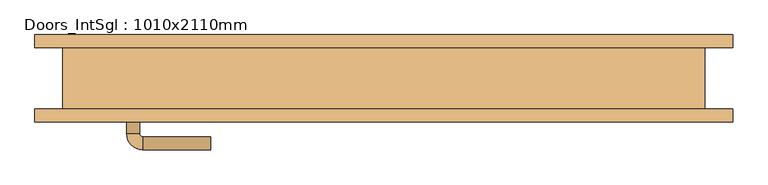
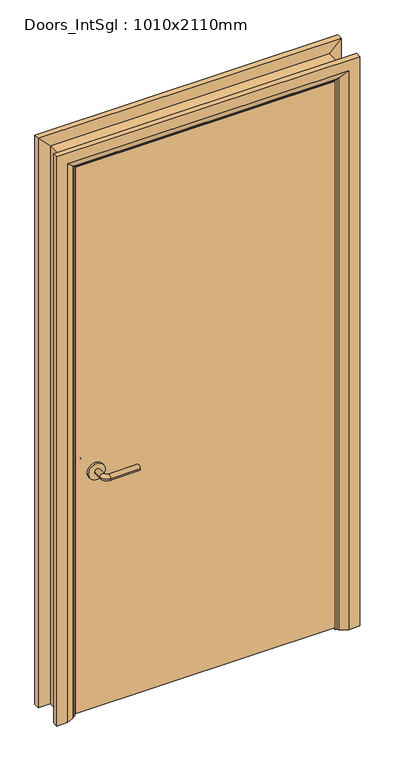
"""IFC4 building model written with IfcOpenShell, lengths in millimetres: door geometry, Doors_IntSgl : 1010x2110mm."""

from ifc_helpers import new_model, si_unit, point, frame, frame_2d, origin, place, context, project, spatial, polyline, circle_curve, ellipse_curve, trimmed, segment, composite_curve, outline, extrude, faceted_brep, source, transform, mapped, element, save
from ifc_brep_helpers import plane_surface, cylinder_surface, revolved_surface, advanced_brep


def doors_intsgl_1010x2110mm_25c8a350(model_context):
    return source(origin(), model_context, "Body", "SolidModel", [
        advanced_brep(
        [(-398.0, -1.5, 900.0), (-378.0, -1.5, 900.0), (-398.0, 28.5, 900.0), (-378.0, 28.5, 900.0), (-373.0, 33.5, 900.0), (-373.0, 53.5, 900.0), (-268.0, 53.5, 900.0), (-268.0, 33.5, 900.0)],
        [
            (0, 1, circle_curve(frame((-388.0, -1.5, 900.0), z_axis=(0.0, -1.0, 0.0), x_axis=(1.0, 0.0, 0.0)), 10.0)),
            (1, 0, circle_curve(frame((-388.0, -1.5, 900.0), z_axis=(0.0, -1.0, 0.0), x_axis=(1.0, 0.0, 0.0)), 10.0)),
            (0, 2),
            (2, 3, circle_curve(frame((-388.0, 28.5, 900.0), z_axis=(0.0, -1.0, 0.0), x_axis=(1.0, 0.0, 0.0)), 10.0)),
            (3, 1),
            (3, 2, circle_curve(frame((-388.0, 28.5, 900.0), z_axis=(0.0, -1.0, 0.0), x_axis=(1.0, 0.0, 0.0)), 10.0)),
            (4, 3, circle_curve(frame((-373.0, 28.5, 900.0), z_axis=(0.0, 0.0, 1.0), x_axis=(-1.0, 0.0, 0.0)), 5.0)),
            (2, 5, circle_curve(frame((-373.0, 28.5, 900.0), z_axis=(0.0, 0.0, -1.0), x_axis=(-1.0, 0.0, 0.0)), 25.0)),
            (5, 4, circle_curve(frame((-373.0, 43.5, 900.0), z_axis=(-1.0, 0.0, 0.0), x_axis=(0.0, -1.0, 0.0)), 10.0)),
            (4, 5, circle_curve(frame((-373.0, 43.5, 900.0), z_axis=(-1.0, 0.0, 0.0), x_axis=(0.0, -1.0, 0.0)), 10.0)),
            (6, 7, circle_curve(frame((-268.0, 43.5, 900.0), z_axis=(1.0, 0.0, 0.0), x_axis=(0.0, -1.0, 0.0)), 10.0)),
            (7, 6, circle_curve(frame((-268.0, 43.5, 900.0), z_axis=(1.0, 0.0, 0.0), x_axis=(0.0, -1.0, 0.0)), 10.0)),
            (5, 6),
            (7, 4),
        ],
        [
            plane_surface(frame((-388.0, -1.5, 900.0), z_axis=(0.0, -1.0, 0.0), x_axis=(0.0, 0.0, 1.0))),
            cylinder_surface(frame((-388.0, -1.5, 900.0), z_axis=(0.0, -1.0, 0.0), x_axis=(1.0, 0.0, 0.0)), 10.0),
            revolved_surface(trimmed(ellipse_curve(frame((-388.0, 28.5, 900.0), z_axis=(0.0, -1.0, 0.0), x_axis=(1.0, 0.0, 0.0)), 10.0, 10.0), [point((-398.0, 28.5, 900.0))], [point((-378.0, 28.5, 900.0))], True, "CARTESIAN"), (-373.0, 28.5, 900.0), (0.0, 0.0, -1.0)),
            revolved_surface(trimmed(ellipse_curve(frame((-388.0, 28.5, 900.0), z_axis=(0.0, -1.0, 0.0), x_axis=(1.0, 0.0, 0.0)), 10.0, 10.0), [point((-378.0, 28.5, 900.0))], [point((-398.0, 28.5, 900.0))], True, "CARTESIAN"), (-373.0, 28.5, 900.0), (0.0, 0.0, -1.0)),
            plane_surface(frame((-268.0, 43.5, 900.0), z_axis=(1.0, 0.0, 0.0), x_axis=(0.0, 0.0, 1.0))),
            cylinder_surface(frame((-373.0, 43.5, 900.0), z_axis=(-1.0, 0.0, 0.0), x_axis=(0.0, -1.0, 0.0)), 10.0),
        ],
        [
            (0, [[1, 2]]),
            (1, [[-1, 3, 4, 5]]),
            (1, [[-2, -5, 6, -3]]),
            (2, [[7, -4, 8, 9]]),
            (3, [[-8, -6, -7, 10]]),
            (4, [[11, 12]]),
            (5, [[-9, 13, -12, 14]]),
            (5, [[-10, -14, -11, -13]]),
        ],
    ),
        extrude(outline(composite_curve([segment(trimmed(circle_curve(frame_2d((900.0, -390.5)), 30.0), [point((900.0, -420.5))], [point((900.0, -360.5))], False, "CARTESIAN"), True, "CONTINUOUS"), segment(trimmed(circle_curve(frame_2d((900.0, -390.5)), 30.0), [point((900.0, -360.5))], [point((900.0, -420.5))], False, "CARTESIAN"), True, "CONTINUOUS")], self_intersect=False)), frame((0.0, -9.5, 0.0), z_axis=(0.0, 1.0, 0.0), x_axis=(0.0, 0.0, 1.0)), (0.0, 0.0, 1.0), 8.0),
        advanced_brep(
        [(-398.0, -55.5, 900.0), (-378.0, -55.5, 900.0), (-378.0, -85.5, 900.0), (-398.0, -85.5, 900.0), (-373.0, -90.5, 900.0), (-373.0, -110.5, 900.0), (-268.0, -110.5, 900.0), (-268.0, -90.5, 900.0)],
        [
            (0, 1, circle_curve(frame((-388.0, -55.5, 900.0), z_axis=(0.0, 1.0, 0.0), x_axis=(1.0, 0.0, 0.0)), 10.0)),
            (1, 0, circle_curve(frame((-388.0, -55.5, 900.0), z_axis=(0.0, 1.0, 0.0), x_axis=(1.0, 0.0, 0.0)), 10.0)),
            (1, 2),
            (2, 3, circle_curve(frame((-388.0, -85.5, 900.0), z_axis=(0.0, 1.0, 0.0), x_axis=(1.0, 0.0, 0.0)), 10.0)),
            (3, 0),
            (3, 2, circle_curve(frame((-388.0, -85.5, 900.0), z_axis=(0.0, 1.0, 0.0), x_axis=(1.0, 0.0, 0.0)), 10.0)),
            (4, 5, circle_curve(frame((-373.0, -100.5, 900.0), z_axis=(-1.0, 0.0, 0.0), x_axis=(0.0, 1.0, 0.0)), 10.0)),
            (5, 3, circle_curve(frame((-373.0, -85.5, 900.0), z_axis=(0.0, 0.0, -1.0), x_axis=(-1.0, 0.0, 0.0)), 25.0)),
            (2, 4, circle_curve(frame((-373.0, -85.5, 900.0), z_axis=(0.0, 0.0, 1.0), x_axis=(-1.0, 0.0, 0.0)), 5.0)),
            (5, 4, circle_curve(frame((-373.0, -100.5, 900.0), z_axis=(-1.0, 0.0, 0.0), x_axis=(0.0, 1.0, 0.0)), 10.0)),
            (6, 7, circle_curve(frame((-268.0, -100.5, 900.0), z_axis=(1.0, 0.0, 0.0), x_axis=(0.0, 1.0, 0.0)), 10.0)),
            (7, 6, circle_curve(frame((-268.0, -100.5, 900.0), z_axis=(1.0, 0.0, 0.0), x_axis=(0.0, 1.0, 0.0)), 10.0)),
            (4, 7),
            (6, 5),
        ],
        [
            plane_surface(frame((-388.0, -55.5, 900.0), z_axis=(0.0, 1.0, 0.0), x_axis=(0.0, 0.0, 1.0))),
            cylinder_surface(frame((-388.0, -55.5, 900.0), z_axis=(0.0, 1.0, 0.0), x_axis=(1.0, 0.0, 0.0)), 10.0),
            revolved_surface(trimmed(ellipse_curve(frame((-388.0, -85.5, 900.0), z_axis=(0.0, -1.0, 0.0), x_axis=(1.0, 0.0, 0.0)), 10.0, 10.0), [point((-398.0, -85.5, 900.0))], [point((-378.0, -85.5, 900.0))], True, "CARTESIAN"), (-373.0, -85.5, 900.0), (0.0, 0.0, -1.0)),
            revolved_surface(trimmed(ellipse_curve(frame((-388.0, -85.5, 900.0), z_axis=(0.0, -1.0, 0.0), x_axis=(1.0, 0.0, 0.0)), 10.0, 10.0), [point((-378.0, -85.5, 900.0))], [point((-398.0, -85.5, 900.0))], True, "CARTESIAN"), (-373.0, -85.5, 900.0), (0.0, 0.0, -1.0)),
            plane_surface(frame((-268.0, -100.5, 900.0), z_axis=(1.0, 0.0, 0.0), x_axis=(0.0, 0.0, 1.0))),
            cylinder_surface(frame((-373.0, -100.5, 900.0), z_axis=(-1.0, 0.0, 0.0), x_axis=(0.0, 1.0, 0.0)), 10.0),
        ],
        [
            (0, [[1, 2]]),
            (1, [[3, 4, 5, -2]]),
            (1, [[-5, 6, -3, -1]]),
            (2, [[7, 8, -4, 9]]),
            (3, [[10, -9, -6, -8]]),
            (4, [[11, 12]]),
            (5, [[13, -11, 14, -7]]),
            (5, [[-14, -12, -13, -10]]),
        ],
    ),
        extrude(outline(composite_curve([segment(trimmed(circle_curve(frame_2d((900.0, -390.5)), 30.0), [point((900.0, -420.5))], [point((900.0, -360.5))], False, "CARTESIAN"), True, "CONTINUOUS"), segment(trimmed(circle_curve(frame_2d((900.0, -390.5)), 30.0), [point((900.0, -360.5))], [point((900.0, -420.5))], False, "CARTESIAN"), True, "CONTINUOUS")], self_intersect=False)), frame((0.0, -55.5, 0.0), z_axis=(0.0, 1.0, 0.0), x_axis=(0.0, 0.0, 1.0)), (0.0, 0.0, 1.0), 8.0),
        extrude(outline(polyline([(463.0, -9.5), (463.0, -47.5), (-463.0, -47.5), (-463.0, -9.5), (463.0, -9.5)])), frame((0.0, 0.0, 8.0), z_axis=(0.0, 0.0, 1.0), x_axis=(1.0, 0.0, 0.0)), (0.0, 0.0, 1.0), 2060.0),
        advanced_brep(
        [(540.0, -67.5, 0.0), (500.0, -67.5, 0.0), (474.0, -53.5, 0.0), (470.0, -47.5, 0.0), (540.0, -47.5, 0.0), (540.0, -47.5, 2145.0), (540.0, -67.5, 2145.0), (470.0, -47.5, 2075.0), (-470.0, -47.5, 2075.0), (-470.0, -47.5, 0.0), (-540.0, -47.5, 0.0), (-540.0, -47.5, 2145.0), (474.0, -53.5, 2079.0), (500.0, -67.5, 2105.0), (-540.0, -67.5, 2145.0), (-540.0, -67.5, 0.0), (-500.0, -67.5, 0.0), (-500.0, -67.5, 2105.0), (-474.0, -53.5, 2079.0), (-474.0, -53.5, 0.0)],
        [
            (0, 1),
            (1, 2),
            (2, 3, circle_curve(frame((478.0, -46.5, 0.0), z_axis=(0.0, 0.0, -1.0), x_axis=(1.0, 0.0, 0.0)), 8.0622577)),
            (3, 4),
            (4, 0),
            (4, 5),
            (5, 6),
            (6, 0),
            (3, 7),
            (7, 8),
            (8, 9),
            (9, 10),
            (10, 11),
            (11, 5),
            (2, 12),
            (12, 7, ellipse_curve(frame((478.0, -46.5, 2083.0), z_axis=(0.7071067811865475, 0.0, -0.7071067811865475), x_axis=(-0.7071067811865474, 0.0, -0.7071067811865476)), 11.4017543, 8.0622577)),
            (1, 13),
            (13, 12),
            (6, 14),
            (14, 15),
            (15, 16),
            (16, 17),
            (17, 13),
            (11, 14),
            (12, 18),
            (18, 8, ellipse_curve(frame((-478.0, -46.5, 2083.0), z_axis=(0.7071067811865475, 0.0, 0.7071067811865475), x_axis=(0.7071067811865476, 0.0, -0.7071067811865474)), 11.4017543, 8.0622577)),
            (17, 18),
            (15, 10),
            (9, 19, circle_curve(frame((-478.0, -46.5, 0.0), z_axis=(0.0, 0.0, -1.0), x_axis=(-1.0, 0.0, 0.0)), 8.0622577)),
            (19, 16),
            (18, 19),
        ],
        [
            plane_surface(frame((470.0, -47.5, 0.0), z_axis=(0.0, 0.0, -1.0), x_axis=(0.0, 1.0, 0.0))),
            plane_surface(frame((540.0, -67.5, 0.0), z_axis=(1.0, 0.0, 0.0), x_axis=(0.0, 0.0, 1.0))),
            plane_surface(frame((540.0, -47.5, 0.0), z_axis=(0.0, 1.0, 0.0), x_axis=(0.0, 0.0, 1.0))),
            cylinder_surface(frame((478.0, -46.5, 0.0), z_axis=(0.0, 0.0, -1.0), x_axis=(1.0, 0.0, 0.0)), 8.0622577),
            plane_surface(frame((474.0, -53.5, 0.0), z_axis=(-0.4740998230350126, -0.880471099922178, 0.0), x_axis=(0.0, 0.0, 1.0))),
            plane_surface(frame((500.0, -67.5, 0.0), z_axis=(0.0, -1.0, 0.0), x_axis=(0.0, 0.0, 1.0))),
            plane_surface(frame((540.0, -67.5, 2145.0), z_axis=(0.0, 0.0, 1.0), x_axis=(-1.0, 0.0, 0.0))),
            cylinder_surface(frame((470.0, -46.5, 2083.0), z_axis=(1.0, 0.0, 0.0), x_axis=(0.0, 0.0, 1.0)), 8.0622577),
            plane_surface(frame((474.0, -53.5, 2079.0), z_axis=(0.0, -0.8804710999221764, -0.4740998230350154), x_axis=(-1.0, 0.0, 0.0))),
            plane_surface(frame((-470.0, -47.5, 0.0), z_axis=(0.0, 0.0, -1.0), x_axis=(0.0, 1.0, 0.0))),
            plane_surface(frame((-540.0, -67.5, 2145.0), z_axis=(-1.0, 0.0, 0.0), x_axis=(0.0, 0.0, -1.0))),
            cylinder_surface(frame((-478.0, -46.5, 2075.0), z_axis=(0.0, 0.0, 1.0), x_axis=(-1.0, 0.0, 0.0)), 8.0622577),
            plane_surface(frame((-474.0, -53.5, 2079.0), z_axis=(0.47409982303501824, -0.8804710999221749, 0.0), x_axis=(0.0, 0.0, -1.0))),
        ],
        [
            (0, [[1, 2, 3, 4, 5]]),
            (1, [[6, 7, 8, -5]]),
            (2, [[9, 10, 11, 12, 13, 14, -6, -4]]),
            (3, [[15, 16, -9, -3]]),
            (4, [[17, 18, -15, -2]]),
            (5, [[-8, 19, 20, 21, 22, 23, -17, -1]]),
            (6, [[-14, 24, -19, -7]]),
            (7, [[25, 26, -10, -16]]),
            (8, [[-23, 27, -25, -18]]),
            (9, [[28, -12, 29, 30, -21]]),
            (10, [[-13, -28, -20, -24]]),
            (11, [[31, -29, -11, -26]]),
            (12, [[-22, -30, -31, -27]]),
        ],
    ),
        extrude(outline(polyline([(0.0, -446.0), (2051.0, -446.0), (2051.0, 446.0), (0.0, 446.0), (0.0, 465.0), (2070.0, 465.0), (2070.0, -465.0), (0.0, -465.0), (0.0, -446.0)])), frame((0.0, -7.5, 0.0), z_axis=(0.0, 1.0, 0.0), x_axis=(0.0, 0.0, 1.0)), (0.0, 0.0, 1.0), 32.0),
        advanced_brep(
        [(-540.0, 67.5, 0.0), (-500.0, 67.5, 0.0), (-474.0, 53.5, 0.0), (-470.0, 47.5, 0.0), (-540.0, 47.5, 0.0), (-540.0, 47.5, 2145.0), (-540.0, 67.5, 2145.0), (-470.0, 47.5, 2075.0), (-474.0, 53.5, 2079.0), (-500.0, 67.5, 2105.0), (540.0, 47.5, 2145.0), (540.0, 67.5, 2145.0), (470.0, 47.5, 2075.0), (474.0, 53.5, 2079.0), (500.0, 67.5, 2105.0), (540.0, 67.5, 0.0), (540.0, 47.5, 0.0), (470.0, 47.5, 0.0), (474.0, 53.5, 0.0), (500.0, 67.5, 0.0)],
        [
            (0, 1),
            (1, 2),
            (2, 3, circle_curve(frame((-478.0, 46.5, 0.0), z_axis=(0.0, 0.0, -1.0), x_axis=(-1.0, 0.0, 0.0)), 8.0622577)),
            (3, 4),
            (4, 0),
            (4, 5),
            (5, 6),
            (6, 0),
            (3, 7),
            (7, 5),
            (2, 8),
            (8, 7, ellipse_curve(frame((-478.0, 46.5, 2083.0), z_axis=(-0.7071067811865475, 0.0, -0.7071067811865475), x_axis=(0.7071067811865474, 0.0, -0.7071067811865476)), 11.4017543, 8.0622577)),
            (1, 9),
            (9, 8),
            (6, 9),
            (5, 10),
            (10, 11),
            (11, 6),
            (7, 12),
            (12, 10),
            (8, 13),
            (13, 12, ellipse_curve(frame((478.0, 46.5, 2083.0), z_axis=(-0.7071067811865475, 0.0, 0.7071067811865475), x_axis=(-0.7071067811865476, 0.0, -0.7071067811865474)), 11.4017543, 8.0622577)),
            (9, 14),
            (14, 13),
            (11, 14),
            (15, 16),
            (16, 17),
            (17, 18, circle_curve(frame((478.0, 46.5, 0.0), z_axis=(0.0, 0.0, -1.0), x_axis=(1.0, 0.0, 0.0)), 8.0622577)),
            (18, 19),
            (19, 15),
            (10, 16),
            (15, 11),
            (12, 17),
            (13, 18),
            (14, 19),
        ],
        [
            plane_surface(frame((-470.0, 120.3010989, 0.0), z_axis=(0.0, 0.0, -1.0), x_axis=(1.0, 0.0, 0.0))),
            plane_surface(frame((-540.0, 67.5, 0.0), z_axis=(-1.0, 0.0, 0.0), x_axis=(0.0, 0.0, 1.0))),
            plane_surface(frame((-540.0, 47.5, 0.0), z_axis=(0.0, -1.0, 0.0), x_axis=(0.0, 0.0, 1.0))),
            cylinder_surface(frame((-478.0, 46.5, 0.0), z_axis=(0.0, 0.0, -1.0), x_axis=(-1.0, 0.0, 0.0)), 8.0622577),
            plane_surface(frame((-474.0, 53.5, 0.0), z_axis=(0.4740998230350183, 0.8804710999221749, 0.0), x_axis=(0.0, 0.0, 1.0))),
            plane_surface(frame((-500.0, 67.5, 0.0), z_axis=(0.0, 1.0, 0.0), x_axis=(0.0, 0.0, 1.0))),
            plane_surface(frame((-540.0, 67.5, 2145.0), z_axis=(0.0, 0.0, 1.0), x_axis=(1.0, 0.0, 0.0))),
            plane_surface(frame((-540.0, 47.5, 2145.0), z_axis=(0.0, -1.0, 0.0), x_axis=(1.0, 0.0, 0.0))),
            cylinder_surface(frame((-470.0, 46.5, 2083.0), z_axis=(-1.0, 0.0, 0.0), x_axis=(0.0, 0.0, 1.0)), 8.0622577),
            plane_surface(frame((-474.0, 53.5, 2079.0), z_axis=(0.0, 0.8804710999221749, -0.4740998230350183), x_axis=(1.0, 0.0, 0.0))),
            plane_surface(frame((-500.0, 67.5, 2105.0), z_axis=(0.0, 1.0, 0.0), x_axis=(1.0, 0.0, 0.0))),
            plane_surface(frame((470.0, 120.3010989, 0.0), z_axis=(0.0, 0.0, -1.0), x_axis=(-1.0, 0.0, 0.0))),
            plane_surface(frame((540.0, 67.5, 2145.0), z_axis=(1.0, 0.0, 0.0), x_axis=(0.0, 0.0, -1.0))),
            plane_surface(frame((540.0, 47.5, 2145.0), z_axis=(0.0, -1.0, 0.0), x_axis=(0.0, 0.0, -1.0))),
            cylinder_surface(frame((478.0, 46.5, 2075.0), z_axis=(0.0, 0.0, 1.0), x_axis=(1.0, 0.0, 0.0)), 8.0622577),
            plane_surface(frame((474.0, 53.5, 2079.0), z_axis=(-0.4740998230350183, 0.8804710999221749, 0.0), x_axis=(0.0, 0.0, -1.0))),
            plane_surface(frame((500.0, 67.5, 2105.0), z_axis=(0.0, 1.0, 0.0), x_axis=(0.0, 0.0, -1.0))),
        ],
        [
            (0, [[1, 2, 3, 4, 5]]),
            (1, [[6, 7, 8, -5]]),
            (2, [[9, 10, -6, -4]]),
            (3, [[11, 12, -9, -3]]),
            (4, [[13, 14, -11, -2]]),
            (5, [[-8, 15, -13, -1]]),
            (6, [[16, 17, 18, -7]]),
            (7, [[19, 20, -16, -10]]),
            (8, [[21, 22, -19, -12]]),
            (9, [[23, 24, -21, -14]]),
            (10, [[-18, 25, -23, -15]]),
            (11, [[26, 27, 28, 29, 30]]),
            (12, [[31, -26, 32, -17]]),
            (13, [[33, -27, -31, -20]]),
            (14, [[34, -28, -33, -22]]),
            (15, [[35, -29, -34, -24]]),
            (16, [[-32, -30, -35, -25]]),
        ],
    ),
        faceted_brep([(-465.0, -47.5, 0.0), (-497.0, -47.5, 0.0), (-497.0, 47.5, 0.0), (-465.0, 47.5, 0.0), (-465.0, 47.5, 2070.0), (-465.0, -47.5, 2070.0), (-497.0, 47.5, 2102.0), (-497.0, -47.5, 2102.0), (465.0, 47.5, 2070.0), (465.0, -47.5, 2070.0), (497.0, 47.5, 2102.0), (497.0, -47.5, 2102.0), (465.0, -47.5, 0.0), (465.0, 47.5, 0.0), (497.0, 47.5, 0.0), (497.0, -47.5, 0.0)], [[[0, 1, 2, 3]], [[3, 4, 5, 0]], [[2, 6, 4, 3]], [[1, 7, 6, 2]], [[0, 5, 7, 1]], [[4, 8, 9, 5]], [[6, 10, 8, 4]], [[7, 11, 10, 6]], [[5, 9, 11, 7]], [[12, 13, 14, 15]], [[8, 13, 12, 9]], [[10, 14, 13, 8]], [[11, 15, 14, 10]], [[9, 12, 15, 11]]]),
    ])


if __name__ == "__main__":
    model = new_model("IFC4")
    model_context = context("Model", 3, world=origin())
    ifc_project = project(units=[si_unit("LENGTHUNIT", "METRE", prefix="MILLI")], contexts=[model_context])
    site = spatial("IfcSite", under=ifc_project)
    building = spatial("IfcBuilding", under=site)
    placement = place(None, origin())
    doors_intsgl_1010x2110mm_shape = doors_intsgl_1010x2110mm_25c8a350(model_context)
    element("IfcDoor", 1, ObjectType="Doors_IntSgl : 1010x2110mm", at=placement, inside=building, context=model_context, shape_type="MappedRepresentation", body=[
        mapped(doors_intsgl_1010x2110mm_shape, transform((0.0, 0.0, 0.0), x_axis=(1.0, 0.0, 0.0), y_axis=(0.0, 1.0, 0.0), z_axis=(0.0, 0.0, 1.0))),
    ])
    save(model, "model.ifc")

# Revit data of these elements
# Type "Doors_IntSgl : 1010x2110mm"
#   Construction Type Id = "MDOOR"
#   Type Mark = "43"
#   Type Comments = "Internal Single"
#   Operation = "SingleSwingRight"
#   Manufacturer = "Revit"
#   Keynote = "L20"
#   Description = "Internal Single Door"
#   Analytic Construction = "Metal"
#   UnderCut = 8 mm
#   Tolerance = 2 mm
#   Thickness = 38 mm
#   Thermal Resistance (R) = 0.270117 (m²·K)/W
#   Structural Tolerance = 8 mm
#   StopDepth = 32 mm
#   Stop Thickness = 19 mm
#   Rough Width = 1010 mm
#   Rough Height = 2110 mm
#   Height to Top Lock Rail = 1000 mm
#   Heat Transfer Coefficient (U) = 3.7021 W/(m²·K)
#   Handle Z Distance = 900 mm
#   Handle X Distance = 75 mm
#   Frame Thickness = 32 mm
#   Door Panel Width = 926 mm
#   Door Panel Thickness = 38 mm
#   Door Panel Offset = 0 mm
#   Height = 2110 mm
#   Width = 1010 mm
#   Door Panel Height = 2060 mm
#   Architrave Setback = 5 mm
#   Vis - Ironmongery = yes
#   Material Ironmongery = Door - Handle
#   Material Frame = Door - Frame/Mullion (1)
#   Material Door = Door - Panel
#   Material Architrave = Door - Architrave
#   Visual Light Transmittance = 0
#   Solar Heat Gain Coefficient = 0
#   Function = (empty or 0)
#   Wall Closure = (empty or 0)
# Element 1 (IfcDoor, "Doors_IntSgl : 1010x2110mm")
#   Materials on its faces: "Door - Architrave", "Door - Handle", "Door - Frame/Mullion (1)", "Door - Panel"
# Materials
#   "Door - Handle": class "Miscellaneous", colour RGB 0 0 0, transparency 0, Keynote = "P21", Cost = 0
#   "Door - Frame/Mullion (1)": class "Wood", colour RGB 212 179 113, transparency 0, Keynote = "L20", Cost = 0
#   "Door - Panel": class "Wood", colour RGB 210 159 95, transparency 0, Keynote = "L20", Cost = 0
#   "Door - Architrave": class "Wood", colour RGB 154 90 5, transparency 0, Keynote = "P20", Cost = 0
